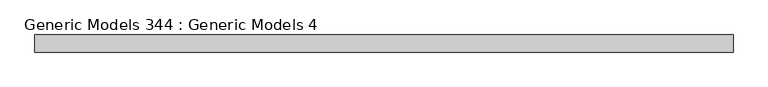
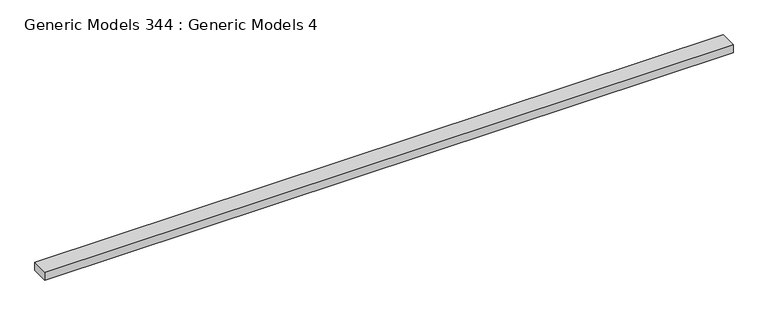
"""IFC4 building model written with IfcOpenShell, lengths in millimetres: proxy geometry, Generic Models 344 : Generic Models 4."""

from ifc_helpers import new_model, si_unit, frame, origin, place, context, project, spatial, polyline, outline, extrude, source, transform, mapped, element, save


def generic_models_344_generic_models_4_9f6bdf57(model_context):
    return source(origin(), model_context, "Body", "SweptSolid", [
        extrude(outline(polyline([(8409.0828684, 7411.5293547), (8409.0828684, 6954.3293547), (-10234.5171316, 6954.3293547), (-10234.5171316, 7411.5293547), (8409.0828684, 7411.5293547)])), frame((0.0, 0.0, 126565.8501918), z_axis=(0.0, 0.0, 1.0), x_axis=(1.0, 0.0, 0.0)), (0.0, 0.0, 1.0), 228.6),
    ])


if __name__ == "__main__":
    model = new_model("IFC4")
    model_context = context("Model", 3, world=origin())
    ifc_project = project(units=[si_unit("LENGTHUNIT", "METRE", prefix="MILLI")], contexts=[model_context])
    site = spatial("IfcSite", under=ifc_project)
    building = spatial("IfcBuilding", under=site)
    placement = place(None, origin())
    generic_models_344_generic_models_4_shape = generic_models_344_generic_models_4_9f6bdf57(model_context)
    element("IfcBuildingElementProxy", 1, Name="Generic Models 344 : Generic Models 4", ObjectType="Generic Models 344 : Generic Models 4", at=placement, inside=building, context=model_context, shape_type="MappedRepresentation", body=[
        mapped(generic_models_344_generic_models_4_shape, transform((0.0, 0.0, 0.0), x_axis=(1.0, 0.0, 0.0), y_axis=(0.0, 1.0, 0.0), z_axis=(0.0, 0.0, 1.0))),
    ])
    save(model, "model.ifc")

# Revit data of these elements
# Element 1 (IfcBuildingElementProxy, "Generic Models 344 : Generic Models 4")
#   Materials on its faces: "_BATT INSUL. (R-FACTOR = R38 MIN) OVER CLASS II VAPOR RETARDER(TOWARD INTERIOR)"
# Materials
#   "_BATT INSUL. (R-FACTOR = R38 MIN) OVER CLASS II VAPOR RETARDER(TOWARD INTERIOR)": class "Generic", colour RGB 227 210 251, transparency 0, Cost = 0
